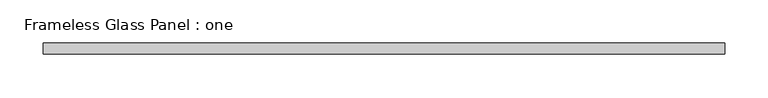
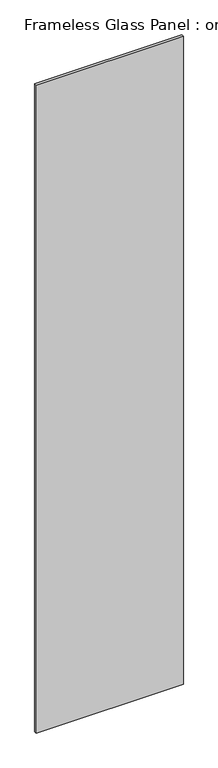
"""IFC4 building model written with IfcOpenShell, lengths in millimetres: plate geometry, Frameless Glass Panel : one."""

from ifc_helpers import new_model, si_unit, origin, origin_with_axes, place, context, project, spatial, polyline, outline, extrude, source, transform, mapped, element, save


def frameless_glass_panel_one_842d672b(model_context):
    return source(origin(), model_context, "Body", "SweptSolid", [
        extrude(outline(polyline([(392.3795501, -6.35), (-392.3795501, -6.35), (-392.3795501, 6.35), (392.3795501, 6.35), (392.3795501, -6.35)])), origin_with_axes(), (0.0, 0.0, 1.0), 3651.25),
    ])


if __name__ == "__main__":
    model = new_model("IFC4")
    model_context = context("Model", 3, world=origin())
    ifc_project = project(units=[si_unit("LENGTHUNIT", "METRE", prefix="MILLI")], contexts=[model_context])
    site = spatial("IfcSite", under=ifc_project)
    building = spatial("IfcBuilding", under=site)
    placement = place(None, origin())
    frameless_glass_panel_one_shape = frameless_glass_panel_one_842d672b(model_context)
    element("IfcPlate", 1, ObjectType="Frameless Glass Panel : one", at=placement, inside=building, context=model_context, shape_type="MappedRepresentation", body=[
        mapped(frameless_glass_panel_one_shape, transform((0.0, 0.0, 0.0), x_axis=(1.0, 0.0, 0.0), y_axis=(0.0, 1.0, 0.0), z_axis=(0.0, 0.0, 1.0))),
    ])
    save(model, "model.ifc")

# Revit data of these elements
# Type "Frameless Glass Panel : one"
#   Glass Thickness = 0' - 0 1/2"
#   Gap btwn Panels = 0' - 0 1/4"
#   Panel Material = TEMPERED GLASS DOOR/SIDELIGHT TO MATCH EXISTING CONF. ROOM
# Element 1 (IfcPlate, "Frameless Glass Panel : one")
#   Materials on its faces: "TEMPERED GLASS DOOR/SIDELIGHT TO MATCH EXISTING CONF. ROOM"
# Materials
#   "TEMPERED GLASS DOOR/SIDELIGHT TO MATCH EXISTING CONF. ROOM": class "Glass", colour RGB 218 227 224, transparency 0.85, Description = "Soda Lime Glass", Cost = 0
